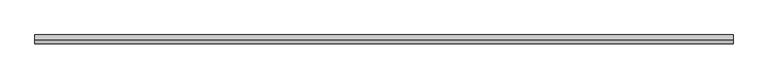
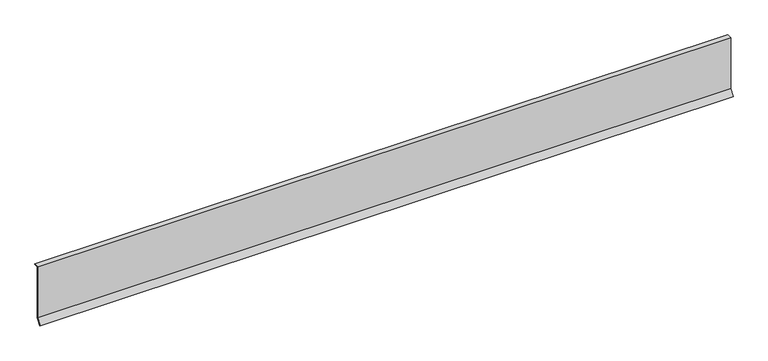
"""IFC4 building model written with IfcOpenShell, lengths in millimetres: proxy geometry, GRAVEL STOP001 34577 : GRAVEL STOP001 34577."""

from ifc_helpers import new_model, si_unit, frame, origin, place, context, project, spatial, polyline, outline, extrude, source, transform, mapped, element, save


def generic_models_6aa894b6(model_context):
    return source(origin(), model_context, "Body", "SweptSolid", [
        extrude(outline(polyline([(-5588.2594715, 40065.903984), (-5575.6959005, 40081.6491197), (-5575.6959005, 40238.3989826), (-5562.5168708, 40238.3989826), (-5562.5168708, 40236.9878716), (-5574.2847895, 40236.9878716), (-5574.2847895, 40081.1551279), (-5587.1564679, 40065.0238605), (-5588.2594715, 40065.903984)])), frame((12382.7678845, 0.0, 0.0), z_axis=(1.0, 0.0, 0.0), x_axis=(0.0, 1.0, 0.0)), (0.0, 0.0, 1.0), 2000.25),
    ])


if __name__ == "__main__":
    model = new_model("IFC4")
    model_context = context("Model", 3, world=origin())
    ifc_project = project(units=[si_unit("LENGTHUNIT", "METRE", prefix="MILLI")], contexts=[model_context])
    site = spatial("IfcSite", under=ifc_project)
    building = spatial("IfcBuilding", under=site)
    placement = place(None, origin())
    generic_models_shape = generic_models_6aa894b6(model_context)
    element("IfcBuildingElementProxy", 1, Name="GRAVEL STOP001 34577 : GRAVEL STOP001 34577", ObjectType="GRAVEL STOP001 34577 : GRAVEL STOP001 34577", at=placement, inside=building, context=model_context, shape_type="MappedRepresentation", body=[
        mapped(generic_models_shape, transform((0.0, 0.0, 0.0), x_axis=(1.0, 0.0, 0.0), y_axis=(0.0, 1.0, 0.0), z_axis=(0.0, 0.0, 1.0))),
    ])
    save(model, "model.ifc")

# Revit data of these elements
# Type "GRAVEL STOP001 34577 : GRAVEL STOP001 34577"
#   NameOverride = "GRAVEL STOP001"
# Element 1 (IfcBuildingElementProxy, "GRAVEL STOP001 34577 : GRAVEL STOP001 34577")
#   Materials on its faces: "GRAVEL STOP REQUIRED WITH GRAVEL SURFACE SYSTEMS"
# Materials
#   "GRAVEL STOP REQUIRED WITH GRAVEL SURFACE SYSTEMS": class "Unassigned", colour RGB 170 170 127, transparency 0
